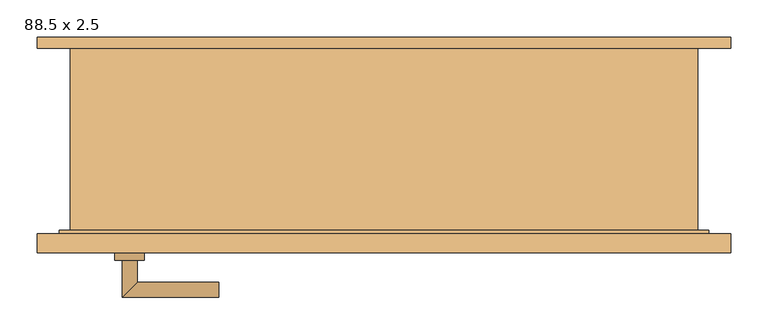
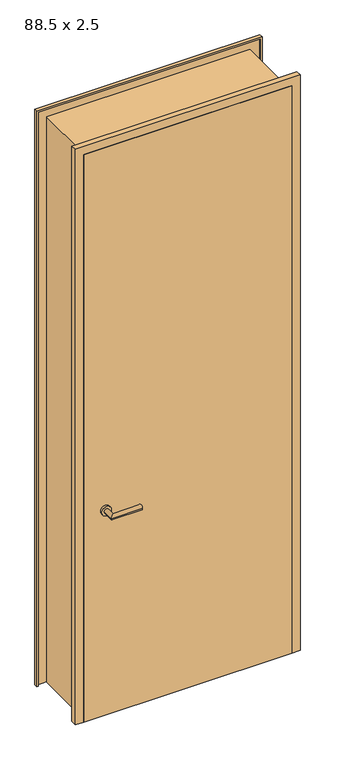
"""IFC4 building model written with IfcOpenShell, lengths in millimetres: door geometry, Drehflügel 1-flg - Stahlzarge : 88.5 x 2.5."""

import ifcopenshell
import ifcopenshell.guid

model = None  # the IFC model being written
_history = None  # IfcOwnerHistory: only IFC2X3 demands one
_inside = {}  # id of a spatial element -> (the spatial element, [elements in it])
_under = {}  # id of a project, library or spatial element -> (it, [spatial elements below it])
_declared = {}  # id of a project -> (the project, [libraries it declares])
_typed = {}  # id of a type object -> (the type object, [elements of that type])
_made_of = {}  # id of a material, layer set ... -> (it, [elements and type objects made of it])


def new_model(schema):
    """Start an empty IFC model of exactly this schema.

    Asked for "IFC4X3", IfcOpenShell would pick the latest addendum, in which some entities
    have other attributes; the version numbers below select the first issue.
    IFC2X3 requires an IfcOwnerHistory on every rooted entity: one is made here for all.
    """
    global model, _history
    if schema == "IFC4X3":
        model = ifcopenshell.file(schema_version=(4, 3, 0, 0))
    else:
        model = ifcopenshell.file(schema=schema)
    _inside.clear()
    _under.clear()
    _declared.clear()
    _typed.clear()
    _made_of.clear()
    _history = None
    if model.schema == "IFC2X3":
        org = make("IfcOrganization", Name="unknown")
        user = make(
            "IfcPersonAndOrganization",
            ThePerson=make("IfcPerson", FamilyName="unknown"),
            TheOrganization=org,
        )
        app = make(
            "IfcApplication",
            ApplicationDeveloper=org,
            Version="unknown",
            ApplicationFullName="unknown",
            ApplicationIdentifier="unknown",
        )
        _history = make(
            "IfcOwnerHistory",
            OwningUser=user,
            OwningApplication=app,
            ChangeAction="ADDED",
            CreationDate=0,
        )
    return model


def make(cls, **values):
    """One entity of the class cls with the attributes given. An attribute that is None is left unset."""
    return model.create_entity(
        cls, **{name: value for name, value in values.items() if value is not None}
    )


def rooted(cls, **values):
    """An entity with a GlobalId (a new one), such as an element, a storey or a relation."""
    return make(cls, GlobalId=ifcopenshell.guid.new(), OwnerHistory=_history, **values)


def si_unit(unit_type, name, prefix=None):
    """IfcSIUnit, for example si_unit("LENGTHUNIT", "METRE", prefix="MILLI")."""
    return make("IfcSIUnit", UnitType=unit_type, Prefix=prefix, Name=name)


def assignment(units):
    """IfcUnitAssignment: the units of a project."""
    return None if units is None else make("IfcUnitAssignment", Units=units)


def point(xyz):
    """IfcCartesianPoint."""
    return None if xyz is None else make("IfcCartesianPoint", Coordinates=xyz)


def direction(xyz):
    """IfcDirection."""
    return None if xyz is None else make("IfcDirection", DirectionRatios=xyz)


def frame(location, z_axis=None, x_axis=None):
    """IfcAxis2Placement3D, a coordinate frame: its origin and axes. An axis left out is left unset."""
    return make(
        "IfcAxis2Placement3D",
        Location=point(location),
        Axis=direction(z_axis),
        RefDirection=direction(x_axis),
    )


def frame_2d(location, x_axis=None):
    """IfcAxis2Placement2D, a coordinate frame in the plane: its origin and x axis."""
    return make(
        "IfcAxis2Placement2D", Location=point(location), RefDirection=direction(x_axis)
    )


def origin():
    """The frame at (0, 0, 0) with its axes left unset."""
    return frame((0.0, 0.0, 0.0))


def place(relative_to, where):
    """IfcLocalPlacement: puts the frame where relative to a parent placement (None: the world)."""
    return make(
        "IfcLocalPlacement", PlacementRelTo=relative_to, RelativePlacement=where
    )


def context(
    kind, dimensions, precision=None, world=None, true_north=None, identifier=None
):
    """IfcGeometricRepresentationContext, for example the 3D "Model" context."""
    return make(
        "IfcGeometricRepresentationContext",
        ContextIdentifier=identifier,
        ContextType=kind,
        CoordinateSpaceDimension=dimensions,
        Precision=precision,
        WorldCoordinateSystem=world,
        TrueNorth=true_north,
    )


def project(units=None, contexts=None):
    """IfcProject with its units and contexts."""
    return rooted(
        "IfcProject",
        Name="project",
        RepresentationContexts=contexts,
        UnitsInContext=assignment(units),
    )


def spatial(cls, under=None, at=None, **own):
    """A site, building, storey or space (cls), placed at a placement, below another one or the project."""
    s = rooted(cls, ObjectPlacement=at, **own)
    if under is not None:
        _under.setdefault(under.id(), (under, []))[1].append(s)
    return s


def polyline(points):
    """IfcPolyline through the points."""
    return make("IfcPolyline", Points=[point(p) for p in points])


def circle_curve(where, radius):
    """IfcCircle in the frame where."""
    return make("IfcCircle", Position=where, Radius=radius)


def ellipse_curve(where, semi_axis1, semi_axis2):
    """IfcEllipse in the frame where."""
    return make(
        "IfcEllipse", Position=where, SemiAxis1=semi_axis1, SemiAxis2=semi_axis2
    )


def trimmed(basis, trim1, trim2, sense, master):
    """IfcTrimmedCurve: the piece of a basis curve between two trims."""
    return make(
        "IfcTrimmedCurve",
        BasisCurve=basis,
        Trim1=trim1,
        Trim2=trim2,
        SenseAgreement=sense,
        MasterRepresentation=master,
    )


def segment(curve, same_sense, transition):
    """IfcCompositeCurveSegment."""
    return make(
        "IfcCompositeCurveSegment",
        Transition=transition,
        SameSense=same_sense,
        ParentCurve=curve,
    )


def composite_curve(segments, self_intersect=None):
    """IfcCompositeCurve: segments joined end to end."""
    return make("IfcCompositeCurve", Segments=segments, SelfIntersect=self_intersect)


def outline(outer, holes=None, kind="AREA"):
    """IfcArbitraryClosedProfileDef: a profile drawn as a closed curve; with holes, ...WithVoids."""
    if holes is None:
        return make("IfcArbitraryClosedProfileDef", ProfileType=kind, OuterCurve=outer)
    return make(
        "IfcArbitraryProfileDefWithVoids",
        ProfileType=kind,
        OuterCurve=outer,
        InnerCurves=holes,
    )


def extrude(swept, where, along, depth):
    """IfcExtrudedAreaSolid: the profile swept, set in the frame where, extruded along a direction by depth."""
    return make(
        "IfcExtrudedAreaSolid",
        SweptArea=swept,
        Position=where,
        ExtrudedDirection=direction(along),
        Depth=depth,
    )


def faces_of(points, faces, orient=None, outer=None):
    """IfcFace entities. A face is a list of loops; a loop is a list of indices into points, from 0.

    orient and outer hold one flag for each loop. By default every Orientation is true, the
    first loop of a face is its IfcFaceOuterBound and the others are IfcFaceBound.
    """
    made = []
    for i, loops in enumerate(faces):
        bounds = []
        for j, loop in enumerate(loops):
            is_outer = j == 0 if outer is None else outer[i][j]
            bounds.append(
                make(
                    "IfcFaceOuterBound" if is_outer else "IfcFaceBound",
                    Bound=make("IfcPolyLoop", Polygon=[points[k] for k in loop]),
                    Orientation=True if orient is None else orient[i][j],
                )
            )
        made.append(make("IfcFace", Bounds=bounds))
    return made


def faceted_brep(points, faces, orient=None, outer=None, voids=None):
    """IfcFacetedBrep: a solid bounded by flat faces; with voids (closed shells), ...WithVoids."""
    shared = [point(p) for p in points]
    hull = make("IfcClosedShell", CfsFaces=faces_of(shared, faces, orient, outer))
    if voids is None:
        return make("IfcFacetedBrep", Outer=hull)
    return make(
        "IfcFacetedBrepWithVoids",
        Outer=hull,
        Voids=[
            make(cls, CfsFaces=faces_of(shared, fs, o, b)) for cls, fs, o, b in voids
        ],
    )


def shape(context_of_items, identifier, shape_type, items):
    """IfcShapeRepresentation: the items that make up one representation, for example the "Body"."""
    return make(
        "IfcShapeRepresentation",
        ContextOfItems=context_of_items,
        RepresentationIdentifier=identifier,
        RepresentationType=shape_type,
        Items=items,
    )


def source(mapping_origin, context_of_items, identifier, shape_type, items):
    """IfcRepresentationMap: a shape defined once, which mapped items show again and again."""
    return make(
        "IfcRepresentationMap",
        MappingOrigin=mapping_origin,
        MappedRepresentation=shape(context_of_items, identifier, shape_type, items),
    )


def transform(
    local_origin,
    x_axis=None,
    y_axis=None,
    z_axis=None,
    scale=None,
    scale2=None,
    scale3=None,
    uniform=True,
):
    """IfcCartesianTransformationOperator3D, or its non-uniform kind. x_axis, y_axis, z_axis: its Axis1, 2, 3."""
    if uniform:
        return make(
            "IfcCartesianTransformationOperator3D",
            Axis1=direction(x_axis),
            Axis2=direction(y_axis),
            LocalOrigin=point(local_origin),
            Scale=scale,
            Axis3=direction(z_axis),
        )
    return make(
        "IfcCartesianTransformationOperator3DnonUniform",
        Axis1=direction(x_axis),
        Axis2=direction(y_axis),
        LocalOrigin=point(local_origin),
        Scale=scale,
        Axis3=direction(z_axis),
        Scale2=scale2,
        Scale3=scale3,
    )


def mapped(mapping_source, mapping_target):
    """IfcMappedItem: shows the shape of a source again, moved by a transform."""
    return make(
        "IfcMappedItem", MappingSource=mapping_source, MappingTarget=mapping_target
    )


def made_of(thing, what):
    """Note that an element or type object is made of a material, layer set ...; save() writes the relation."""
    if what is not None:
        _made_of.setdefault(what.id(), (what, []))[1].append(thing)
    return thing


def element(
    cls,
    number,
    at=None,
    inside=None,
    cuts=None,
    type_object=None,
    material=None,
    context=None,
    identifier="Body",
    shape_type=None,
    held_by="IfcProductDefinitionShape",
    body=None,
    shapes=None,
    **own,
):
    """One element of the class cls, such as IfcWall. Its Tag is "e" and its number.

    at: its placement. inside: the storey or other place that contains it. cuts: it is an
    opening in that element (IfcRelVoidsElement). A single representation is given by context,
    identifier, shape_type and body (its items); several are given by shapes. held_by: the class
    of the entity that holds the representations. save() writes the other relations.
    """
    e = rooted(cls, Tag="e%d" % number, ObjectPlacement=at, **own)
    if body is not None:
        shapes = [shape(context, identifier, shape_type, body)]
    if shapes is not None:
        e.Representation = make(held_by, Representations=shapes)
    if inside is not None:
        _inside.setdefault(inside.id(), (inside, []))[1].append(e)
    if cuts is not None:
        rooted(
            "IfcRelVoidsElement", RelatingBuildingElement=cuts, RelatedOpeningElement=e
        )
    if type_object is not None:
        _typed.setdefault(type_object.id(), (type_object, []))[1].append(e)
    return made_of(e, material)


def aggregate(whole, parts):
    """IfcRelAggregates: a whole, such as a stair, and the parts it consists of."""
    return rooted("IfcRelAggregates", RelatingObject=whole, RelatedObjects=parts)


def save(model, path):
    """Write the relations noted so far, then the file.

    IfcRelAggregates (storeys below a building ...), IfcRelContainedInSpatialStructure (elements
    in a storey), IfcRelDefinesByType, IfcRelAssociatesMaterial and IfcRelDeclares: one each for
    every whole, place, type object, material and project.
    """
    for whole, parts in _under.values():
        aggregate(whole, parts)
    for where, things in _inside.values():
        rooted(
            "IfcRelContainedInSpatialStructure",
            RelatedElements=things,
            RelatingStructure=where,
        )
    for kind, things in _typed.values():
        rooted("IfcRelDefinesByType", RelatedObjects=things, RelatingType=kind)
    for what, things in _made_of.values():
        rooted("IfcRelAssociatesMaterial", RelatedObjects=things, RelatingMaterial=what)
    for by, libraries in _declared.values():
        rooted("IfcRelDeclares", RelatingContext=by, RelatedDefinitions=libraries)
    model.write(path)


def plane_surface(at):
    """IfcPlane: the flat surface through the origin of the frame at, square to its z axis."""
    return make("IfcPlane", Position=at)


def cylinder_surface(at, radius):
    """IfcCylindricalSurface: all points at the distance radius from the z axis of the frame at."""
    return make("IfcCylindricalSurface", Position=at, Radius=radius)


def advanced_brep(points, edges, surfaces, faces):
    """IfcAdvancedBrep: a solid bounded by faces that lie on surfaces and meet in shared edges.

    An edge is (start, end): straight between two places in points (the first is 0);
    or (start, end, curve); or (start, end, curve, False) where it runs against its curve.
    A face is (place in surfaces, loops), or (place, loops, False) where it looks against
    its surface's normal. A loop lists edges by number (the first is 1), with a minus sign
    where the edge is run from its end to its start. The first loop is the outer one.
    """
    corners = [point(p) for p in points]
    vertices = [make("IfcVertexPoint", VertexGeometry=c) for c in corners]
    made = []
    for start, end, *more in edges:
        made.append(
            make(
                "IfcEdgeCurve",
                EdgeStart=vertices[start],
                EdgeEnd=vertices[end],
                EdgeGeometry=more[0] if more else make("IfcPolyline", Points=[corners[start], corners[end]]),
                SameSense=more[1] if len(more) > 1 else True,
            )
        )
    hull = []
    for where, loops, *sense in faces:
        bounds = []
        for j, loop in enumerate(loops):
            ring = [make("IfcOrientedEdge", EdgeElement=made[abs(k) - 1], Orientation=k > 0) for k in loop]
            bounds.append(
                make(
                    "IfcFaceOuterBound" if j == 0 else "IfcFaceBound",
                    Bound=make("IfcEdgeLoop", EdgeList=ring),
                    Orientation=True,
                )
            )
        hull.append(make("IfcAdvancedFace", Bounds=bounds, FaceSurface=surfaces[where], SameSense=sense[0] if sense else True))
    return make("IfcAdvancedBrep", Outer=make("IfcClosedShell", CfsFaces=hull))


def door_88_5_x_2_5_7381d536(model_context):
    return source(origin(), model_context, "Body", "SolidModel", [
        advanced_brep(
        [(-352.5, -114.4346141, 901.0), (-332.5, -114.4346141, 901.0), (-332.5, -64.4346141, 901.0), (-352.5, -44.4346141, 901.0), (-222.5, -44.4346141, 901.0), (-222.5, -64.4346141, 901.0)],
        [
            (0, 1, circle_curve(frame((-342.5, -114.4346141, 901.0), z_axis=(0.0, -1.0, 0.0), x_axis=(1.0, 0.0, 0.0)), 10.0)),
            (1, 0, circle_curve(frame((-342.5, -114.4346141, 901.0), z_axis=(0.0, -1.0, 0.0), x_axis=(1.0, 0.0, 0.0)), 10.0)),
            (1, 2),
            (2, 3, ellipse_curve(frame((-342.5, -54.4346141, 901.0), z_axis=(-0.7071067811865385, -0.7071067811865565, 0.0), x_axis=(0.7071067811865563, -0.7071067811865386, 0.0)), 14.1421356, 10.0)),
            (3, 0),
            (3, 2, ellipse_curve(frame((-342.5, -54.4346141, 901.0), z_axis=(-0.7071067811865385, -0.7071067811865565, 0.0), x_axis=(0.7071067811865563, -0.7071067811865386, 0.0)), 14.1421356, 10.0)),
            (4, 5, circle_curve(frame((-222.5, -54.4346141, 901.0), z_axis=(1.0, 0.0, 0.0), x_axis=(0.0, -1.0, 0.0)), 10.0)),
            (5, 4, circle_curve(frame((-222.5, -54.4346141, 901.0), z_axis=(1.0, 0.0, 0.0), x_axis=(0.0, -1.0, 0.0)), 10.0)),
            (2, 5),
            (4, 3),
        ],
        [
            plane_surface(frame((-342.5, -114.4346141, -386.7526403), z_axis=(0.0, -1.0, 0.0), x_axis=(0.0, 0.0, 1.0))),
            cylinder_surface(frame((-342.5, -114.4346141, 901.0), z_axis=(0.0, -1.0, 0.0), x_axis=(1.0, 0.0, 0.0)), 10.0),
            plane_surface(frame((-222.5, -54.4346141, -386.7526403), z_axis=(1.0, 0.0, 0.0), x_axis=(0.0, 0.0, 1.0))),
            cylinder_surface(frame((-342.5, -54.4346141, 901.0), z_axis=(-1.0, 0.0, 0.0), x_axis=(0.0, -1.0, 0.0)), 10.0),
        ],
        [
            (0, [[1, 2]]),
            (1, [[3, 4, 5, -2]]),
            (1, [[-5, 6, -3, -1]]),
            (2, [[7, 8]]),
            (3, [[9, -7, 10, -4]]),
            (3, [[-10, -8, -9, -6]]),
        ],
    ),
        advanced_brep(
        [(-332.5, -174.4346141, 901.0), (-352.5, -174.4346141, 901.0), (-352.5, -224.4346141, 901.0), (-332.5, -204.4346141, 901.0), (-222.5, -204.4346141, 901.0), (-222.5, -224.4346141, 901.0)],
        [
            (0, 1, circle_curve(frame((-342.5, -174.4346141, 901.0), z_axis=(0.0, 1.0, 0.0), x_axis=(-1.0, 0.0, 0.0)), 10.0)),
            (1, 0, circle_curve(frame((-342.5, -174.4346141, 901.0), z_axis=(0.0, 1.0, 0.0), x_axis=(-1.0, 0.0, 0.0)), 10.0)),
            (1, 2),
            (2, 3, ellipse_curve(frame((-342.5, -214.4346141, 901.0), z_axis=(-0.7071067811865475, 0.7071067811865475, 0.0), x_axis=(0.7071067811865474, 0.7071067811865476, 0.0)), 14.1421356, 10.0)),
            (3, 0),
            (3, 2, ellipse_curve(frame((-342.5, -214.4346141, 901.0), z_axis=(-0.7071067811865475, 0.7071067811865475, 0.0), x_axis=(0.7071067811865474, 0.7071067811865476, 0.0)), 14.1421356, 10.0)),
            (4, 5, circle_curve(frame((-222.5, -214.4346141, 901.0), z_axis=(1.0, 0.0, 0.0), x_axis=(0.0, -1.0, 0.0)), 10.0)),
            (5, 4, circle_curve(frame((-222.5, -214.4346141, 901.0), z_axis=(1.0, 0.0, 0.0), x_axis=(0.0, -1.0, 0.0)), 10.0)),
            (2, 5),
            (4, 3),
        ],
        [
            plane_surface(frame((-342.5, -174.4346141, -386.7526403), z_axis=(0.0, 1.0, 0.0), x_axis=(0.0, 0.0, 1.0))),
            cylinder_surface(frame((-342.5, -174.4346141, 901.0), z_axis=(0.0, 1.0, 0.0), x_axis=(-1.0, 0.0, 0.0)), 10.0),
            plane_surface(frame((-222.5, -214.4346141, -386.7526403), z_axis=(1.0, 0.0, 0.0), x_axis=(0.0, 0.0, 1.0))),
            cylinder_surface(frame((-342.5, -214.4346141, 901.0), z_axis=(-1.0, 0.0, 0.0), x_axis=(0.0, -1.0, 0.0)), 10.0),
        ],
        [
            (0, [[1, 2]]),
            (1, [[3, 4, 5, -2]]),
            (1, [[-5, 6, -3, -1]]),
            (2, [[7, 8]]),
            (3, [[9, -7, 10, -4]]),
            (3, [[-10, -8, -9, -6]]),
        ],
    ),
        extrude(outline(composite_curve([segment(trimmed(circle_curve(frame_2d((901.0, -342.5)), 20.0), [point((901.0, -362.5))], [point((901.0, -322.5))], False, "CARTESIAN"), True, "CONTINUOUS"), segment(trimmed(circle_curve(frame_2d((901.0, -342.5)), 20.0), [point((901.0, -322.5))], [point((901.0, -362.5))], False, "CARTESIAN"), True, "CONTINUOUS")], self_intersect=False)), frame((0.0, -114.4346141, 0.0), z_axis=(0.0, 1.0, 0.0), x_axis=(0.0, 0.0, 1.0)), (0.0, 0.0, 1.0), 10.0),
        extrude(outline(composite_curve([segment(trimmed(circle_curve(frame_2d((901.0, -342.5)), 20.0), [point((901.0, -362.5))], [point((901.0, -322.5))], False, "CARTESIAN"), True, "CONTINUOUS"), segment(trimmed(circle_curve(frame_2d((901.0, -342.5)), 20.0), [point((901.0, -322.5))], [point((901.0, -362.5))], False, "CARTESIAN"), True, "CONTINUOUS")], self_intersect=False)), frame((0.0, -174.4346141, 0.0), z_axis=(0.0, 1.0, 0.0), x_axis=(0.0, 0.0, 1.0)), (0.0, 0.0, 1.0), 10.0),
        extrude(outline(polyline([(432.5, -139.4346141), (432.5, -164.4346141), (-432.5, -164.4346141), (-432.5, -139.4346141), (432.5, -139.4346141)])), frame((0.0, 0.0, 1.0), z_axis=(0.0, 0.0, 1.0), x_axis=(1.0, 0.0, 0.0)), (0.0, 0.0, 1.0), 2490.0),
        faceted_brep([(466.9603207, 125.5653859, 1.0), (466.9603207, 110.5653859, 1.0), (461.9603207, 110.5653859, 1.0), (461.9603207, 120.5653859, 1.0), (422.5, 120.5653859, 1.0), (422.5, -134.4346141, 1.0), (437.5, -134.4346141, 1.0), (437.5, -159.4346141, 1.0), (461.9603207, -159.4346141, 1.0), (461.9603207, -139.4346141, 1.0), (466.9603207, -139.4346141, 1.0), (466.9603207, -164.4346141, 1.0), (432.5, -164.4346141, 1.0), (432.5, -139.4346141, 1.0), (417.5, -139.4346141, 1.0), (417.5, 125.5653859, 1.0), (417.5, 125.5653859, 2476.0), (-417.5, 125.5653859, 2476.0), (-417.5, 125.5653859, 1.0), (-466.9603207, 125.5653859, 1.0), (-466.9603207, 125.5653859, 2525.4603207), (466.9603207, 125.5653859, 2525.4603207), (417.5, -139.4346141, 2476.0), (432.5, -139.4346141, 2491.0), (-432.5, -139.4346141, 2491.0), (-432.5, -139.4346141, 1.0), (-417.5, -139.4346141, 1.0), (-417.5, -139.4346141, 2476.0), (432.5, -164.4346141, 2491.0), (466.9603207, -164.4346141, 2525.4603207), (-466.9603207, -164.4346141, 2525.4603207), (-466.9603207, -164.4346141, 1.0), (-432.5, -164.4346141, 1.0), (-432.5, -164.4346141, 2491.0), (466.9603207, -139.4346141, 2525.4603207), (461.9603207, -139.4346141, 2520.4603207), (-461.9603207, -139.4346141, 2520.4603207), (-461.9603207, -139.4346141, 1.0), (-466.9603207, -139.4346141, 1.0), (-466.9603207, -139.4346141, 2525.4603207), (461.9603207, -159.4346141, 2520.4603207), (437.5, -159.4346141, 2496.0), (-437.5, -159.4346141, 2496.0), (-437.5, -159.4346141, 1.0), (-461.9603207, -159.4346141, 1.0), (-461.9603207, -159.4346141, 2520.4603207), (437.5, -134.4346141, 2496.0), (422.5, -134.4346141, 2481.0), (-422.5, -134.4346141, 2481.0), (-422.5, -134.4346141, 1.0), (-437.5, -134.4346141, 1.0), (-437.5, -134.4346141, 2496.0), (422.5, 120.5653859, 2481.0), (461.9603207, 120.5653859, 2520.4603207), (-461.9603207, 120.5653859, 2520.4603207), (-461.9603207, 120.5653859, 1.0), (-422.5, 120.5653859, 1.0), (-422.5, 120.5653859, 2481.0), (461.9603207, 110.5653859, 2520.4603207), (466.9603207, 110.5653859, 2525.4603207), (-466.9603207, 110.5653859, 2525.4603207), (-466.9603207, 110.5653859, 1.0), (-461.9603207, 110.5653859, 1.0), (-461.9603207, 110.5653859, 2520.4603207)], [[[0, 1, 2, 3, 4, 5, 6, 7, 8, 9, 10, 11, 12, 13, 14, 15]], [[15, 16, 17, 18, 19, 20, 21, 0]], [[14, 22, 16, 15]], [[13, 23, 24, 25, 26, 27, 22, 14]], [[12, 28, 23, 13]], [[11, 29, 30, 31, 32, 33, 28, 12]], [[10, 34, 29, 11]], [[9, 35, 36, 37, 38, 39, 34, 10]], [[8, 40, 35, 9]], [[7, 41, 42, 43, 44, 45, 40, 8]], [[6, 46, 41, 7]], [[5, 47, 48, 49, 50, 51, 46, 6]], [[4, 52, 47, 5]], [[3, 53, 54, 55, 56, 57, 52, 4]], [[2, 58, 53, 3]], [[1, 59, 60, 61, 62, 63, 58, 2]], [[0, 21, 59, 1]], [[20, 19, 61, 60]], [[19, 18, 26, 25, 32, 31, 38, 37, 44, 43, 50, 49, 56, 55, 62, 61]], [[27, 26, 18, 17]], [[33, 32, 25, 24]], [[39, 38, 31, 30]], [[45, 44, 37, 36]], [[51, 50, 43, 42]], [[57, 56, 49, 48]], [[63, 62, 55, 54]], [[22, 27, 17, 16]], [[28, 33, 24, 23]], [[34, 39, 30, 29]], [[40, 45, 36, 35]], [[46, 51, 42, 41]], [[52, 57, 48, 47]], [[58, 63, 54, 53]], [[21, 20, 60, 59]]]),
    ])


if __name__ == "__main__":
    model = new_model("IFC4")
    model_context = context("Model", 3, world=origin())
    ifc_project = project(units=[si_unit("LENGTHUNIT", "METRE", prefix="MILLI")], contexts=[model_context])
    site = spatial("IfcSite", under=ifc_project)
    building = spatial("IfcBuilding", under=site)
    placement = place(None, origin())
    door_88_5_x_2_5_shape = door_88_5_x_2_5_7381d536(model_context)
    element("IfcDoor", 1, ObjectType="Drehflügel 1-flg - Stahlzarge : 88.5 x 2.5", at=placement, inside=building, context=model_context, shape_type="MappedRepresentation", body=[
        mapped(door_88_5_x_2_5_shape, transform((0.0, 0.0, 0.0), x_axis=(1.0, 0.0, 0.0), y_axis=(0.0, 1.0, 0.0), z_axis=(0.0, 0.0, 1.0))),
    ])
    save(model, "model.ifc")

# Revit data of these elements
# Type "Drehflügel 1-flg - Stahlzarge : 88.5 x 2.5"
#   Type Mark = "22"
#   Operation = "SingleSwingRight"
#   Keynote = "16.03"
#   Analytic Construction = "Metall"
#   Thermal Resistance (R) = 0.270117 (m²·K)/W
#   Heat Transfer Coefficient (U) = 3.7021 W/(m²·K)
#   Rough Width = 0.885 m
#   Rough Height [instance default] = 2.600 m
#   Höhe Türgriff [instance default] = 0.900 m
#   Height = 2.500 m
#   Fußbodenaufbau [instance default] = 0.100 m
#   Width = 0.885 m
#   Sichtbarkeit Sturzlinien [instance default] = yes
#   Türgriff auswählen [instance default] = element 221079
#   Türgriff [instance default] = none
#   Türflügel [instance default] = none
#   Rahmen/Pfosten [instance default] = Metall - Lackiert - Grau
#   Visual Light Transmittance = 0
#   Solar Heat Gain Coefficient = 0
#   Function = (empty or 0)
#   Wall Closure = (empty or 0)
# Element 1 (IfcDoor, "Drehflügel 1-flg - Stahlzarge : 88.5 x 2.5")
#   Rough Height = 2.501 m
#   Fußbodenaufbau = 0.001 m
#   Materials on its faces: "Metall - Lackiert - Grau", "Metall - Chrom", "Holz - Birke"
# Materials
#   "Metall - Lackiert - Grau": class "Farbe 1", colour RGB 98 98 98, transparency 0, Cost = 0
#   "Metall - Chrom": class "Metall", colour RGB 247 247 247, transparency 0, Cost = 0
#   "Holz - Birke": class "Holz", colour RGB 213 164 103, transparency 0, Cost = 0
